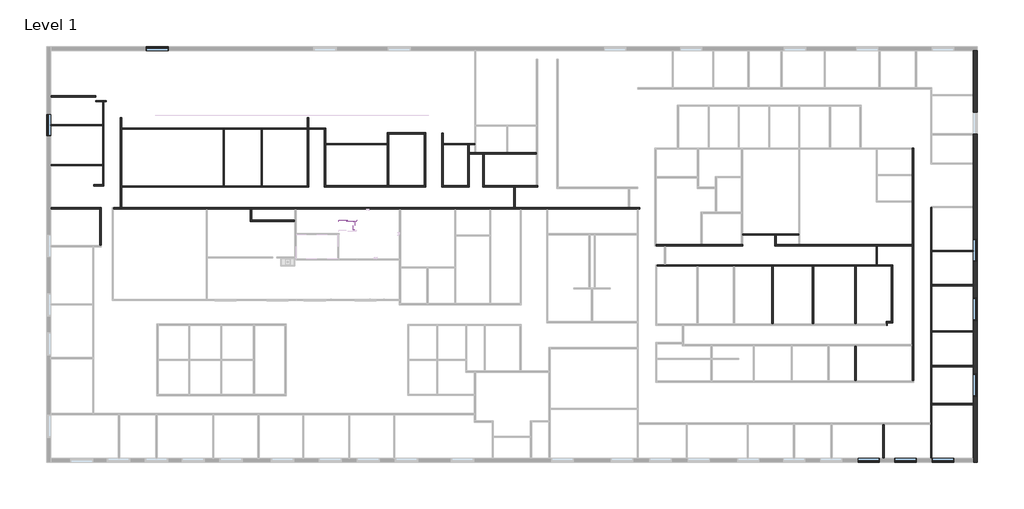
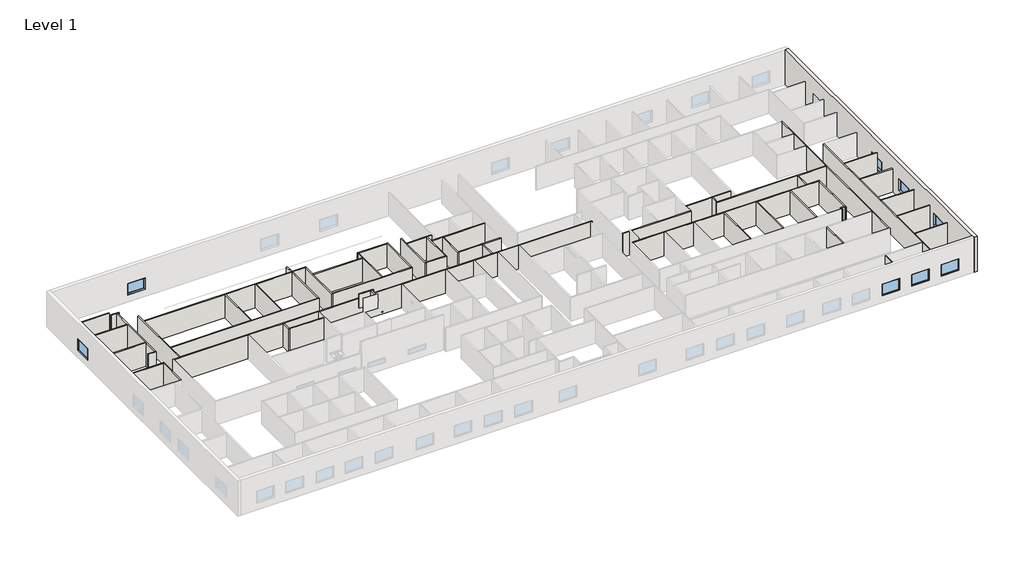
# One storey, part 3 of 4: 55 walls, 8 windows.
"""IFC4 building model written with IfcOpenShell, lengths in millimetres."""

import ifcopenshell
import ifcopenshell.guid

model = None  # the IFC model being written
_history = None  # IfcOwnerHistory: only IFC2X3 demands one
_inside = {}  # id of a spatial element -> (the spatial element, [elements in it])
_under = {}  # id of a project, library or spatial element -> (it, [spatial elements below it])
_declared = {}  # id of a project -> (the project, [libraries it declares])
_typed = {}  # id of a type object -> (the type object, [elements of that type])
_made_of = {}  # id of a material, layer set ... -> (it, [elements and type objects made of it])


def new_model(schema):
    """Start an empty IFC model of exactly this schema.

    Asked for "IFC4X3", IfcOpenShell would pick the latest addendum, in which some entities
    have other attributes; the version numbers below select the first issue.
    IFC2X3 requires an IfcOwnerHistory on every rooted entity: one is made here for all.
    """
    global model, _history
    if schema == "IFC4X3":
        model = ifcopenshell.file(schema_version=(4, 3, 0, 0))
    else:
        model = ifcopenshell.file(schema=schema)
    _inside.clear()
    _under.clear()
    _declared.clear()
    _typed.clear()
    _made_of.clear()
    _history = None
    if model.schema == "IFC2X3":
        org = make("IfcOrganization", Name="unknown")
        user = make(
            "IfcPersonAndOrganization",
            ThePerson=make("IfcPerson", FamilyName="unknown"),
            TheOrganization=org,
        )
        app = make(
            "IfcApplication",
            ApplicationDeveloper=org,
            Version="unknown",
            ApplicationFullName="unknown",
            ApplicationIdentifier="unknown",
        )
        _history = make(
            "IfcOwnerHistory",
            OwningUser=user,
            OwningApplication=app,
            ChangeAction="ADDED",
            CreationDate=0,
        )
    return model


def make(cls, **values):
    """One entity of the class cls with the attributes given. An attribute that is None is left unset."""
    return model.create_entity(
        cls, **{name: value for name, value in values.items() if value is not None}
    )


def rooted(cls, **values):
    """An entity with a GlobalId (a new one), such as an element, a storey or a relation."""
    return make(cls, GlobalId=ifcopenshell.guid.new(), OwnerHistory=_history, **values)


def si_unit(unit_type, name, prefix=None):
    """IfcSIUnit, for example si_unit("LENGTHUNIT", "METRE", prefix="MILLI")."""
    return make("IfcSIUnit", UnitType=unit_type, Prefix=prefix, Name=name)


def assignment(units):
    """IfcUnitAssignment: the units of a project."""
    return None if units is None else make("IfcUnitAssignment", Units=units)


def point(xyz):
    """IfcCartesianPoint."""
    return None if xyz is None else make("IfcCartesianPoint", Coordinates=xyz)


def direction(xyz):
    """IfcDirection."""
    return None if xyz is None else make("IfcDirection", DirectionRatios=xyz)


def frame(location, z_axis=None, x_axis=None):
    """IfcAxis2Placement3D, a coordinate frame: its origin and axes. An axis left out is left unset."""
    return make(
        "IfcAxis2Placement3D",
        Location=point(location),
        Axis=direction(z_axis),
        RefDirection=direction(x_axis),
    )


def origin():
    """The frame at (0, 0, 0) with its axes left unset."""
    return frame((0.0, 0.0, 0.0))


def origin_with_axes():
    """The frame at (0, 0, 0) with the z axis (0, 0, 1) and the x axis (1, 0, 0) written out."""
    return frame((0.0, 0.0, 0.0), z_axis=(0.0, 0.0, 1.0), x_axis=(1.0, 0.0, 0.0))


def place(relative_to, where):
    """IfcLocalPlacement: puts the frame where relative to a parent placement (None: the world)."""
    return make(
        "IfcLocalPlacement", PlacementRelTo=relative_to, RelativePlacement=where
    )


def context(
    kind, dimensions, precision=None, world=None, true_north=None, identifier=None
):
    """IfcGeometricRepresentationContext, for example the 3D "Model" context."""
    return make(
        "IfcGeometricRepresentationContext",
        ContextIdentifier=identifier,
        ContextType=kind,
        CoordinateSpaceDimension=dimensions,
        Precision=precision,
        WorldCoordinateSystem=world,
        TrueNorth=true_north,
    )


def project(units=None, contexts=None):
    """IfcProject with its units and contexts."""
    return rooted(
        "IfcProject",
        Name="project",
        RepresentationContexts=contexts,
        UnitsInContext=assignment(units),
    )


def spatial(cls, under=None, at=None, **own):
    """A site, building, storey or space (cls), placed at a placement, below another one or the project."""
    s = rooted(cls, ObjectPlacement=at, **own)
    if under is not None:
        _under.setdefault(under.id(), (under, []))[1].append(s)
    return s


def polyline(points):
    """IfcPolyline through the points."""
    return make("IfcPolyline", Points=[point(p) for p in points])


def outline(outer, holes=None, kind="AREA"):
    """IfcArbitraryClosedProfileDef: a profile drawn as a closed curve; with holes, ...WithVoids."""
    if holes is None:
        return make("IfcArbitraryClosedProfileDef", ProfileType=kind, OuterCurve=outer)
    return make(
        "IfcArbitraryProfileDefWithVoids",
        ProfileType=kind,
        OuterCurve=outer,
        InnerCurves=holes,
    )


def extrude(swept, where, along, depth):
    """IfcExtrudedAreaSolid: the profile swept, set in the frame where, extruded along a direction by depth."""
    return make(
        "IfcExtrudedAreaSolid",
        SweptArea=swept,
        Position=where,
        ExtrudedDirection=direction(along),
        Depth=depth,
    )


def faces_of(points, faces, orient=None, outer=None):
    """IfcFace entities. A face is a list of loops; a loop is a list of indices into points, from 0.

    orient and outer hold one flag for each loop. By default every Orientation is true, the
    first loop of a face is its IfcFaceOuterBound and the others are IfcFaceBound.
    """
    made = []
    for i, loops in enumerate(faces):
        bounds = []
        for j, loop in enumerate(loops):
            is_outer = j == 0 if outer is None else outer[i][j]
            bounds.append(
                make(
                    "IfcFaceOuterBound" if is_outer else "IfcFaceBound",
                    Bound=make("IfcPolyLoop", Polygon=[points[k] for k in loop]),
                    Orientation=True if orient is None else orient[i][j],
                )
            )
        made.append(make("IfcFace", Bounds=bounds))
    return made


def faceted_brep(points, faces, orient=None, outer=None, voids=None):
    """IfcFacetedBrep: a solid bounded by flat faces; with voids (closed shells), ...WithVoids."""
    shared = [point(p) for p in points]
    hull = make("IfcClosedShell", CfsFaces=faces_of(shared, faces, orient, outer))
    if voids is None:
        return make("IfcFacetedBrep", Outer=hull)
    return make(
        "IfcFacetedBrepWithVoids",
        Outer=hull,
        Voids=[
            make(cls, CfsFaces=faces_of(shared, fs, o, b)) for cls, fs, o, b in voids
        ],
    )


def shape(context_of_items, identifier, shape_type, items):
    """IfcShapeRepresentation: the items that make up one representation, for example the "Body"."""
    return make(
        "IfcShapeRepresentation",
        ContextOfItems=context_of_items,
        RepresentationIdentifier=identifier,
        RepresentationType=shape_type,
        Items=items,
    )


def source(mapping_origin, context_of_items, identifier, shape_type, items):
    """IfcRepresentationMap: a shape defined once, which mapped items show again and again."""
    return make(
        "IfcRepresentationMap",
        MappingOrigin=mapping_origin,
        MappedRepresentation=shape(context_of_items, identifier, shape_type, items),
    )


def transform(
    local_origin,
    x_axis=None,
    y_axis=None,
    z_axis=None,
    scale=None,
    scale2=None,
    scale3=None,
    uniform=True,
):
    """IfcCartesianTransformationOperator3D, or its non-uniform kind. x_axis, y_axis, z_axis: its Axis1, 2, 3."""
    if uniform:
        return make(
            "IfcCartesianTransformationOperator3D",
            Axis1=direction(x_axis),
            Axis2=direction(y_axis),
            LocalOrigin=point(local_origin),
            Scale=scale,
            Axis3=direction(z_axis),
        )
    return make(
        "IfcCartesianTransformationOperator3DnonUniform",
        Axis1=direction(x_axis),
        Axis2=direction(y_axis),
        LocalOrigin=point(local_origin),
        Scale=scale,
        Axis3=direction(z_axis),
        Scale2=scale2,
        Scale3=scale3,
    )


def mapped(mapping_source, mapping_target):
    """IfcMappedItem: shows the shape of a source again, moved by a transform."""
    return make(
        "IfcMappedItem", MappingSource=mapping_source, MappingTarget=mapping_target
    )


def made_of(thing, what):
    """Note that an element or type object is made of a material, layer set ...; save() writes the relation."""
    if what is not None:
        _made_of.setdefault(what.id(), (what, []))[1].append(thing)
    return thing


def element(
    cls,
    number,
    at=None,
    inside=None,
    cuts=None,
    type_object=None,
    material=None,
    context=None,
    identifier="Body",
    shape_type=None,
    held_by="IfcProductDefinitionShape",
    body=None,
    shapes=None,
    **own,
):
    """One element of the class cls, such as IfcWall. Its Tag is "e" and its number.

    at: its placement. inside: the storey or other place that contains it. cuts: it is an
    opening in that element (IfcRelVoidsElement). A single representation is given by context,
    identifier, shape_type and body (its items); several are given by shapes. held_by: the class
    of the entity that holds the representations. save() writes the other relations.
    """
    e = rooted(cls, Tag="e%d" % number, ObjectPlacement=at, **own)
    if body is not None:
        shapes = [shape(context, identifier, shape_type, body)]
    if shapes is not None:
        e.Representation = make(held_by, Representations=shapes)
    if inside is not None:
        _inside.setdefault(inside.id(), (inside, []))[1].append(e)
    if cuts is not None:
        rooted(
            "IfcRelVoidsElement", RelatingBuildingElement=cuts, RelatedOpeningElement=e
        )
    if type_object is not None:
        _typed.setdefault(type_object.id(), (type_object, []))[1].append(e)
    return made_of(e, material)


def aggregate(whole, parts):
    """IfcRelAggregates: a whole, such as a stair, and the parts it consists of."""
    return rooted("IfcRelAggregates", RelatingObject=whole, RelatedObjects=parts)


def save(model, path):
    """Write the relations noted so far, then the file.

    IfcRelAggregates (storeys below a building ...), IfcRelContainedInSpatialStructure (elements
    in a storey), IfcRelDefinesByType, IfcRelAssociatesMaterial and IfcRelDeclares: one each for
    every whole, place, type object, material and project.
    """
    for whole, parts in _under.values():
        aggregate(whole, parts)
    for where, things in _inside.values():
        rooted(
            "IfcRelContainedInSpatialStructure",
            RelatedElements=things,
            RelatingStructure=where,
        )
    for kind, things in _typed.values():
        rooted("IfcRelDefinesByType", RelatedObjects=things, RelatingType=kind)
    for what, things in _made_of.values():
        rooted("IfcRelAssociatesMaterial", RelatedObjects=things, RelatingMaterial=what)
    for by, libraries in _declared.values():
        rooted("IfcRelDeclares", RelatingContext=by, RelatedDefinitions=libraries)
    model.write(path)


def window_d56d71bd(model_context):
    return source(origin(), model_context, "Body", "SweptSolid", [
        extrude(outline(polyline([(990.6, 50.8), (-1066.8, 50.8), (-1066.8, 63.5), (990.6, 63.5), (990.6, 50.8)])), frame((0.0, 0.0, 977.9), z_axis=(0.0, 0.0, 1.0), x_axis=(1.0, 0.0, 0.0)), (0.0, 0.0, 1.0), 1397.0),
        extrude(outline(polyline([(2419.35, -1111.25), (933.45, -1111.25), (933.45, 1035.05), (2419.35, 1035.05), (2419.35, -1111.25)]), holes=[polyline([(2374.9, -1066.8), (2374.9, 990.6), (977.9, 990.6), (977.9, -1066.8), (2374.9, -1066.8)])]), frame((0.0, 34.925, 0.0), z_axis=(0.0, 1.0, 0.0), x_axis=(0.0, 0.0, 1.0)), (0.0, 0.0, 1.0), 44.45),
        extrude(outline(polyline([(2438.4, -1130.3), (914.4, -1130.3), (914.4, 1054.1), (2438.4, 1054.1), (2438.4, -1130.3)]), holes=[polyline([(2406.65, -1098.55), (2406.65, 1022.35), (946.15, 1022.35), (946.15, -1098.55), (2406.65, -1098.55)])]), frame((0.0, -206.375, 0.0), z_axis=(0.0, 1.0, 0.0), x_axis=(0.0, 0.0, 1.0)), (0.0, 0.0, 1.0), 241.3),
        extrude(outline(polyline([(2438.4, 1054.1), (2438.4, -1130.3), (914.4, -1130.3), (914.4, 1054.1), (2438.4, 1054.1)]), holes=[polyline([(2419.35, 1035.05), (933.45, 1035.05), (933.45, -1111.25), (2419.35, -1111.25), (2419.35, 1035.05)])]), frame((0.0, 34.925, 0.0), z_axis=(0.0, 1.0, 0.0), x_axis=(0.0, 0.0, 1.0)), (0.0, 0.0, 1.0), 171.45),
    ])


model = new_model("IFC4")

# Units and contexts
model_context = context("Model", 3, world=origin())
ifc_project = project(units=[si_unit("LENGTHUNIT", "METRE", prefix="MILLI")], contexts=[model_context])

# Site, building, storey
site = spatial("IfcSite", under=ifc_project)
building = spatial("IfcBuilding", under=site)
storey = spatial("IfcBuildingStorey", under=building, Name="Level 1", Elevation=0.0)

# Walls
placement = place(None, origin())
element("IfcWall", 1, ObjectType="Exterior Wall", at=placement, inside=storey, context=model_context, shape_type="Brep", body=[
    faceted_brep([(139716.6178914, 17535.8048706, 0.0), (139716.6178914, 6497.9173706, 0.0), (139716.6178914, 6374.0923706, 0.0), (139716.6178914, -22532.6951294, 0.0), (139716.6178914, -22945.4451294, 0.0), (139716.6178914, -22945.4451294, 4572.0), (139716.6178914, -22532.6951294, 4572.0), (139716.6178914, 17535.8048706, 4572.0), (139716.6178914, -16439.8701294, 2438.4), (139716.6178914, -16439.8701294, 914.4), (139716.6178914, -14255.4701294, 914.4), (139716.6178914, -14255.4701294, 2438.4), (139716.6178914, -8972.2701294, 2438.4), (139716.6178914, -8972.2701294, 914.4), (139716.6178914, -6787.8701294, 914.4), (139716.6178914, -6787.8701294, 2438.4), (139716.6178914, -3181.0701294, 2438.4), (139716.6178914, -3181.0701294, 914.4), (139716.6178914, -996.6701294, 914.4), (139716.6178914, -996.6701294, 2438.4), (139716.6178914, 9309.3798706, 2438.4), (139716.6178914, 9309.3798706, 914.4), (139716.6178914, 11493.7798706, 914.4), (139716.6178914, 11493.7798706, 2438.4), (140129.3678914, -22945.4451294, 0.0), (140129.3678914, 17535.8048706, 0.0), (140129.3678914, 17535.8048706, 4572.0), (140129.3678914, -22945.4451294, 4572.0), (140129.3678914, -16439.8701294, 914.4), (140129.3678914, -16439.8701294, 2438.4), (140129.3678914, -14255.4701294, 2438.4), (140129.3678914, -14255.4701294, 914.4), (140129.3678914, -8972.2701294, 914.4), (140129.3678914, -8972.2701294, 2438.4), (140129.3678914, -6787.8701294, 2438.4), (140129.3678914, -6787.8701294, 914.4), (140129.3678914, -3181.0701294, 914.4), (140129.3678914, -3181.0701294, 2438.4), (140129.3678914, -996.6701294, 2438.4), (140129.3678914, -996.6701294, 914.4), (140129.3678914, 9309.3798706, 914.4), (140129.3678914, 9309.3798706, 2438.4), (140129.3678914, 11493.7798706, 2438.4), (140129.3678914, 11493.7798706, 914.4)], [[[0, 1, 2, 3, 4, 5, 6, 7], [8, 9, 10, 11], [12, 13, 14, 15], [16, 17, 18, 19], [20, 21, 22, 23]], [[24, 25, 26, 27], [28, 29, 30, 31], [32, 33, 34, 35], [36, 37, 38, 39], [40, 41, 42, 43]], [[4, 3, 2, 1, 0, 25, 24]], [[7, 6, 5, 27, 26]], [[0, 7, 26, 25]], [[5, 4, 24, 27]], [[8, 29, 28, 9]], [[9, 28, 31, 10]], [[10, 31, 30, 11]], [[29, 8, 11, 30]], [[12, 33, 32, 13]], [[13, 32, 35, 14]], [[14, 35, 34, 15]], [[33, 12, 15, 34]], [[16, 37, 36, 17]], [[17, 36, 39, 18]], [[18, 39, 38, 19]], [[37, 16, 19, 38]], [[20, 41, 40, 21]], [[21, 40, 43, 22]], [[22, 43, 42, 23]], [[41, 20, 23, 42]]]),
])
element("IfcWall", 2, ObjectType="Interior - 4 7/8\" Partition (1-hr)", at=placement, inside=storey, context=model_context, shape_type="Brep", body=[
    faceted_brep([(54053.4683253, -1628.1381812, 0.0), (54053.4683253, 2105.6618188, 0.0), (54053.4683253, 2105.6618188, 3048.0), (54053.4683253, -1628.1381812, 3048.0), (53929.6433253, 2105.6618188, 0.0), (53929.6433253, 1981.8368188, 0.0), (53929.6433253, -1628.1381812, 0.0), (53929.6433253, -1628.1381812, 3048.0), (53929.6433253, 1981.8368188, 3048.0), (53929.6433253, 2105.6618188, 3048.0)], [[[0, 1, 2, 3]], [[4, 5, 6, 7, 8, 9]], [[1, 0, 6, 5, 4]], [[3, 2, 9, 8, 7]], [[0, 3, 7, 6]], [[2, 1, 4, 9]]]),
])
element("IfcWall", 3, ObjectType="Interior - 4 7/8\" Partition (1-hr)", at=placement, inside=storey, context=model_context, shape_type="SweptSolid", body=[
    extrude(outline(polyline([(49102.1178914, 2105.6618188), (53929.6433253, 2105.6618188), (53929.6433253, 1981.8368188), (49102.1178914, 1981.8368188), (49102.1178914, 2105.6618188)])), origin_with_axes(), (0.0, 0.0, 1.0), 3048.0),
])
element("IfcWall", 4, ObjectType="Interior - 4 7/8\" Partition (1-hr)", at=placement, inside=storey, context=model_context, shape_type="Brep", body=[
    faceted_brep([(55252.655131, 1981.8368188, 0.0), (64363.2514852, 1981.8368188, 0.0), (64487.0764852, 1981.8368188, 0.0), (68717.830131, 1981.8368188, 0.0), (68841.655131, 1981.8368188, 0.0), (73075.4514852, 1981.8368188, 0.0), (73199.2764852, 1981.8368188, 0.0), (83337.0514852, 1981.8368188, 0.0), (83460.8764852, 1981.8368188, 0.0), (95198.8514852, 1981.8368188, 0.0), (95322.6764852, 1981.8368188, 0.0), (106944.7639852, 1981.8368188, 0.0), (106944.7639852, 1981.8368188, 3048.0), (95322.6764852, 1981.8368188, 3048.0), (95198.8514852, 1981.8368188, 3048.0), (83460.8764852, 1981.8368188, 3048.0), (83337.0514852, 1981.8368188, 3048.0), (73199.2764852, 1981.8368188, 3048.0), (73075.4514852, 1981.8368188, 3048.0), (68841.655131, 1981.8368188, 3048.0), (68717.830131, 1981.8368188, 3048.0), (64487.0764852, 1981.8368188, 3048.0), (64363.2514852, 1981.8368188, 3048.0), (55252.655131, 1981.8368188, 3048.0), (106944.7639852, 2105.6618188, 0.0), (56065.455131, 2105.6618188, 0.0), (55941.630131, 2105.6618188, 0.0), (55252.655131, 2105.6618188, 0.0), (55252.655131, 2105.6618188, 3048.0), (55941.630131, 2105.6618188, 3048.0), (56065.455131, 2105.6618188, 3048.0), (106944.7639852, 2105.6618188, 3048.0)], [[[0, 1, 2, 3, 4, 5, 6, 7, 8, 9, 10, 11, 12, 13, 14, 15, 16, 17, 18, 19, 20, 21, 22, 23]], [[24, 25, 26, 27, 28, 29, 30, 31]], [[11, 10, 9, 8, 7, 6, 5, 4, 3, 2, 1, 0, 27, 26, 25, 24]], [[12, 11, 24, 31]], [[23, 22, 21, 20, 19, 18, 17, 16, 15, 14, 13, 12, 31, 30, 29, 28]], [[0, 23, 28, 27]]]),
])
element("IfcWall", 5, ObjectType="Interior - 4 7/8\" Partition (1-hr)", at=placement, inside=storey, context=model_context, shape_type="Brep", body=[
    faceted_brep([(54320.2303914, 4363.6075038, 0.0), (54320.2303914, 12510.9870321, 0.0), (54320.2303914, 12510.9870321, 3048.0), (54320.2303914, 4363.6075038, 3048.0), (54196.4053914, 12510.9870321, 0.0), (54196.4053914, 10272.6120321, 0.0), (54196.4053914, 10148.7870321, 0.0), (54196.4053914, 6345.9759689, 0.0), (54196.4053914, 6222.1509689, 0.0), (54196.4053914, 4363.6075038, 0.0), (54196.4053914, 4363.6075038, 3048.0), (54196.4053914, 6222.1509689, 3048.0), (54196.4053914, 6345.9759689, 3048.0), (54196.4053914, 10148.7870321, 3048.0), (54196.4053914, 10272.6120321, 3048.0), (54196.4053914, 12510.9870321, 3048.0)], [[[0, 1, 2, 3]], [[4, 5, 6, 7, 8, 9, 10, 11, 12, 13, 14, 15]], [[1, 0, 9, 8, 7, 6, 5, 4]], [[3, 2, 15, 14, 13, 12, 11, 10]], [[0, 3, 10, 9]], [[2, 1, 4, 15]]]),
])
element("IfcWall", 6, ObjectType="Interior - 4 7/8\" Partition (1-hr)", at=placement, inside=storey, context=model_context, shape_type="Brep", body=[
    faceted_brep([(54559.8105998, 12634.8120321, 0.0), (53543.8105998, 12634.8120321, 0.0), (53543.8105998, 12634.8120321, 3048.0), (54559.8105998, 12634.8120321, 3048.0), (54559.8105998, 12510.9870321, 0.0), (54559.8105998, 12510.9870321, 3048.0), (54320.2303914, 12510.9870321, 3048.0), (54196.4053914, 12510.9870321, 3048.0), (53543.8105998, 12510.9870321, 3048.0), (53543.8105998, 12510.9870321, 0.0), (54196.4053914, 12510.9870321, 0.0), (54320.2303914, 12510.9870321, 0.0)], [[[0, 1, 2, 3]], [[4, 5, 6, 7, 8, 9, 10, 11]], [[1, 0, 4, 11, 10, 9]], [[2, 1, 9, 8]], [[3, 2, 8, 7, 6, 5]], [[0, 3, 5, 4]]]),
])
element("IfcWall", 7, ObjectType="Interior - 4 7/8\" Partition (1-hr)", at=placement, inside=storey, context=model_context, shape_type="SweptSolid", body=[
    extrude(outline(polyline([(49102.1178914, 13092.0120321), (53543.8105998, 13092.0120321), (53543.8105998, 12968.1870321), (49102.1178914, 12968.1870321), (49102.1178914, 13092.0120321)])), origin_with_axes(), (0.0, 0.0, 1.0), 3048.0),
])
element("IfcWall", 8, ObjectType="Interior - 4 7/8\" Partition (1-hr)", at=placement, inside=storey, context=model_context, shape_type="SweptSolid", body=[
    extrude(outline(polyline([(49102.1178914, 10272.6120321), (54196.4053914, 10272.6120321), (54196.4053914, 10148.7870321), (49102.1178914, 10148.7870321), (49102.1178914, 10272.6120321)])), origin_with_axes(), (0.0, 0.0, 1.0), 3048.0),
])
element("IfcWall", 9, ObjectType="Interior - 4 7/8\" Partition (1-hr)", at=placement, inside=storey, context=model_context, shape_type="SweptSolid", body=[
    extrude(outline(polyline([(49102.1178914, 6345.9759689), (54196.4053914, 6345.9759689), (54196.4053914, 6222.1509689), (49102.1178914, 6222.1509689), (49102.1178914, 6345.9759689)])), origin_with_axes(), (0.0, 0.0, 1.0), 3048.0),
])
element("IfcWall", 10, ObjectType="Interior - 4 7/8\" Partition (1-hr)", at=placement, inside=storey, context=model_context, shape_type="Brep", body=[
    faceted_brep([(56065.455131, 2105.6618188, 0.0), (56065.455131, 4115.4368188, 0.0), (56065.455131, 4239.2618188, 0.0), (56065.455131, 9818.5870321, 0.0), (56065.455131, 9942.4120321, 0.0), (56065.455131, 10964.580131, 0.0), (56065.455131, 10964.580131, 3048.0), (56065.455131, 9942.4120321, 3048.0), (56065.455131, 9818.5870321, 3048.0), (56065.455131, 4239.2618188, 3048.0), (56065.455131, 4115.4368188, 3048.0), (56065.455131, 2105.6618188, 3048.0), (55941.630131, 10964.580131, 0.0), (55941.630131, 2105.6618188, 0.0), (55941.630131, 2105.6618188, 3048.0), (55941.630131, 10964.580131, 3048.0)], [[[0, 1, 2, 3, 4, 5, 6, 7, 8, 9, 10, 11]], [[12, 13, 14, 15]], [[5, 4, 3, 2, 1, 0, 13, 12]], [[6, 5, 12, 15]], [[11, 10, 9, 8, 7, 6, 15, 14]], [[0, 11, 14, 13]]]),
])
element("IfcWall", 11, ObjectType="Interior - 4 7/8\" Partition (1-hr)", at=placement, inside=storey, context=model_context, shape_type="Brep", body=[
    faceted_brep([(56065.455131, 9818.5870321, 0.0), (66025.430131, 9818.5870321, 0.0), (66149.255131, 9818.5870321, 0.0), (69759.230131, 9818.5870321, 0.0), (69883.055131, 9818.5870321, 0.0), (74305.830131, 9818.5870321, 0.0), (74429.655131, 9818.5870321, 0.0), (75982.230131, 9818.5870321, 0.0), (76106.055131, 9818.5870321, 0.0), (76106.055131, 9818.5870321, 3048.0), (75982.230131, 9818.5870321, 3048.0), (74429.655131, 9818.5870321, 3048.0), (74305.830131, 9818.5870321, 3048.0), (69883.055131, 9818.5870321, 3048.0), (69759.230131, 9818.5870321, 3048.0), (66149.255131, 9818.5870321, 3048.0), (66025.430131, 9818.5870321, 3048.0), (56065.455131, 9818.5870321, 3048.0), (76106.055131, 9942.4120321, 0.0), (74429.655131, 9942.4120321, 0.0), (74305.830131, 9942.4120321, 0.0), (56065.455131, 9942.4120321, 0.0), (56065.455131, 9942.4120321, 3048.0), (74305.830131, 9942.4120321, 3048.0), (74429.655131, 9942.4120321, 3048.0), (76106.055131, 9942.4120321, 3048.0)], [[[0, 1, 2, 3, 4, 5, 6, 7, 8, 9, 10, 11, 12, 13, 14, 15, 16, 17]], [[18, 19, 20, 21, 22, 23, 24, 25]], [[8, 7, 6, 5, 4, 3, 2, 1, 0, 21, 20, 19, 18]], [[17, 16, 15, 14, 13, 12, 11, 10, 9, 25, 24, 23, 22]], [[0, 17, 22, 21]], [[9, 8, 18, 25]]]),
])
element("IfcWall", 12, ObjectType="Interior - 4 7/8\" Partition (1-hr)", at=placement, inside=storey, context=model_context, shape_type="Brep", body=[
    faceted_brep([(75982.230131, 9818.5870321, 0.0), (75982.230131, 4129.995756, 0.0), (75982.230131, 4129.995756, 3048.0), (75982.230131, 9818.5870321, 3048.0), (76106.055131, 9818.5870321, 0.0), (76106.055131, 9818.5870321, 3048.0), (76106.055131, 8419.420756, 3048.0), (76106.055131, 8295.595756, 3048.0), (76106.055131, 4253.820756, 3048.0), (76106.055131, 4129.995756, 3048.0), (76106.055131, 4129.995756, 0.0), (76106.055131, 4253.820756, 0.0), (76106.055131, 8295.595756, 0.0), (76106.055131, 8419.420756, 0.0)], [[[0, 1, 2, 3]], [[4, 5, 6, 7, 8, 9, 10, 11, 12, 13]], [[1, 0, 4, 13, 12, 11, 10]], [[3, 2, 9, 8, 7, 6, 5]], [[0, 3, 5, 4]], [[2, 1, 10, 9]]]),
])
element("IfcWall", 13, ObjectType="Interior - 4 7/8\" Partition (1-hr)", at=placement, inside=storey, context=model_context, shape_type="Brep", body=[
    faceted_brep([(76106.055131, 4129.995756, 0.0), (85935.855131, 4129.995756, 0.0), (85935.855131, 4129.995756, 3048.0), (76106.055131, 4129.995756, 3048.0), (85935.855131, 4253.820756, 0.0), (85812.030131, 4253.820756, 0.0), (82303.655131, 4253.820756, 0.0), (82179.830131, 4253.820756, 0.0), (76106.055131, 4253.820756, 0.0), (76106.055131, 4253.820756, 3048.0), (82179.830131, 4253.820756, 3048.0), (82303.655131, 4253.820756, 3048.0), (85812.030131, 4253.820756, 3048.0), (85935.855131, 4253.820756, 3048.0)], [[[0, 1, 2, 3]], [[4, 5, 6, 7, 8, 9, 10, 11, 12, 13]], [[1, 0, 8, 7, 6, 5, 4]], [[3, 2, 13, 12, 11, 10, 9]], [[0, 3, 9, 8]], [[2, 1, 4, 13]]]),
])
element("IfcWall", 14, ObjectType="Interior - 4 7/8\" Partition (1-hr)", at=placement, inside=storey, context=model_context, shape_type="Brep", body=[
    faceted_brep([(85935.855131, 4253.820756, 0.0), (85935.855131, 9460.820756, 0.0), (85935.855131, 9460.820756, 3048.0), (85935.855131, 4253.820756, 3048.0), (85812.030131, 4253.820756, 0.0), (85812.030131, 4253.820756, 3048.0), (85812.030131, 9336.995756, 3048.0), (85812.030131, 9460.820756, 3048.0), (85812.030131, 9460.820756, 0.0), (85812.030131, 9336.995756, 0.0)], [[[0, 1, 2, 3]], [[4, 5, 6, 7, 8, 9]], [[1, 0, 4, 9, 8]], [[3, 2, 7, 6, 5]], [[0, 3, 5, 4]], [[2, 1, 8, 7]]]),
])
element("IfcWall", 15, ObjectType="Interior - 4 7/8\" Partition (1-hr)", at=placement, inside=storey, context=model_context, shape_type="Brep", body=[
    faceted_brep([(85812.030131, 9460.820756, 0.0), (82179.830131, 9460.820756, 0.0), (82179.830131, 9460.820756, 3048.0), (85812.030131, 9460.820756, 3048.0), (82179.830131, 9336.995756, 0.0), (82303.655131, 9336.995756, 0.0), (85812.030131, 9336.995756, 0.0), (85812.030131, 9336.995756, 3048.0), (82303.655131, 9336.995756, 3048.0), (82179.830131, 9336.995756, 3048.0)], [[[0, 1, 2, 3]], [[4, 5, 6, 7, 8, 9]], [[1, 0, 6, 5, 4]], [[3, 2, 9, 8, 7]], [[0, 3, 7, 6]], [[2, 1, 4, 9]]]),
])
element("IfcWall", 16, ObjectType="Interior - 4 7/8\" Partition (1-hr)", at=placement, inside=storey, context=model_context, shape_type="Brep", body=[
    faceted_brep([(82179.830131, 9336.995756, 0.0), (82179.830131, 8419.420756, 0.0), (82179.830131, 8295.595756, 0.0), (82179.830131, 4253.820756, 0.0), (82179.830131, 4253.820756, 3048.0), (82179.830131, 8295.595756, 3048.0), (82179.830131, 8419.420756, 3048.0), (82179.830131, 9336.995756, 3048.0), (82303.655131, 9336.995756, 0.0), (82303.655131, 9336.995756, 3048.0), (82303.655131, 4253.820756, 3048.0), (82303.655131, 4253.820756, 0.0)], [[[0, 1, 2, 3, 4, 5, 6, 7]], [[8, 9, 10, 11]], [[3, 2, 1, 0, 8, 11]], [[7, 6, 5, 4, 10, 9]], [[0, 7, 9, 8]], [[4, 3, 11, 10]]]),
])
element("IfcWall", 17, ObjectType="Interior - 4 7/8\" Partition (1-hr)", at=placement, inside=storey, context=model_context, shape_type="SweptSolid", body=[
    extrude(outline(polyline([(76106.055131, 8419.420756), (82179.830131, 8419.420756), (82179.830131, 8295.595756), (76106.055131, 8295.595756), (76106.055131, 8419.420756)])), origin_with_axes(), (0.0, 0.0, 1.0), 3048.0),
])
element("IfcWall", 18, ObjectType="Interior - 4 7/8\" Partition (1-hr)", at=placement, inside=storey, context=model_context, shape_type="Brep", body=[
    faceted_brep([(87533.1447144, 9438.5296102, 0.0), (87533.1447144, 4129.995756, 0.0), (87533.1447144, 4129.995756, 3048.0), (87533.1447144, 9438.5296102, 3048.0), (87656.9697144, 9438.5296102, 0.0), (87656.9697144, 9438.5296102, 3048.0), (87656.9697144, 8419.420756, 3048.0), (87656.9697144, 8295.595756, 3048.0), (87656.9697144, 4253.820756, 3048.0), (87656.9697144, 4129.995756, 3048.0), (87656.9697144, 4129.995756, 0.0), (87656.9697144, 4253.820756, 0.0), (87656.9697144, 8295.595756, 0.0), (87656.9697144, 8419.420756, 0.0)], [[[0, 1, 2, 3]], [[4, 5, 6, 7, 8, 9, 10, 11, 12, 13]], [[1, 0, 4, 13, 12, 11, 10]], [[3, 2, 9, 8, 7, 6, 5]], [[0, 3, 5, 4]], [[2, 1, 10, 9]]]),
])
element("IfcWall", 19, ObjectType="Interior - 4 7/8\" Partition (1-hr)", at=placement, inside=storey, context=model_context, shape_type="Brep", body=[
    faceted_brep([(87656.9697144, 4129.995756, 0.0), (90196.9697144, 4129.995756, 0.0), (90196.9697144, 4129.995756, 3048.0), (87656.9697144, 4129.995756, 3048.0), (87656.9697144, 4253.820756, 0.0), (87656.9697144, 4253.820756, 3048.0), (90073.1447144, 4253.820756, 3048.0), (90196.9697144, 4253.820756, 3048.0), (90196.9697144, 4253.820756, 0.0), (90073.1447144, 4253.820756, 0.0)], [[[0, 1, 2, 3]], [[4, 5, 6, 7, 8, 9]], [[1, 0, 4, 9, 8]], [[3, 2, 7, 6, 5]], [[0, 3, 5, 4]], [[2, 1, 8, 7]]]),
])
element("IfcWall", 20, ObjectType="Interior - 4 7/8\" Partition (1-hr)", at=placement, inside=storey, context=model_context, shape_type="Brep", body=[
    faceted_brep([(90196.9697144, 4253.820756, 0.0), (90196.9697144, 7390.0923706, 0.0), (90196.9697144, 7513.9173706, 0.0), (90196.9697144, 8295.595756, 0.0), (90196.9697144, 8295.595756, 3048.0), (90196.9697144, 7513.9173706, 3048.0), (90196.9697144, 7390.0923706, 3048.0), (90196.9697144, 4253.820756, 3048.0), (90073.1447144, 4253.820756, 0.0), (90073.1447144, 4253.820756, 3048.0), (90073.1447144, 8295.595756, 3048.0), (90073.1447144, 8295.595756, 0.0)], [[[0, 1, 2, 3, 4, 5, 6, 7]], [[8, 9, 10, 11]], [[3, 2, 1, 0, 8, 11]], [[7, 6, 5, 4, 10, 9]], [[0, 7, 9, 8]], [[4, 3, 11, 10]]]),
])
element("IfcWall", 21, ObjectType="Interior - 4 7/8\" Partition (1-hr)", at=placement, inside=storey, context=model_context, shape_type="Brep", body=[
    faceted_brep([(87656.9697144, 8295.595756, 0.0), (90073.1447144, 8295.595756, 0.0), (90196.9697144, 8295.595756, 0.0), (90729.1866283, 8295.595756, 0.0), (90729.1866283, 8295.595756, 3048.0), (90196.9697144, 8295.595756, 3048.0), (90073.1447144, 8295.595756, 3048.0), (87656.9697144, 8295.595756, 3048.0), (87656.9697144, 8419.420756, 0.0), (87656.9697144, 8419.420756, 3048.0), (90729.1866283, 8419.420756, 3048.0), (90729.1866283, 8419.420756, 0.0)], [[[0, 1, 2, 3, 4, 5, 6, 7]], [[8, 9, 10, 11]], [[3, 2, 1, 0, 8, 11]], [[7, 6, 5, 4, 10, 9]], [[0, 7, 9, 8]], [[4, 3, 11, 10]]]),
])
element("IfcWall", 22, ObjectType="Interior - 4 7/8\" Partition (1-hr)", at=placement, inside=storey, context=model_context, shape_type="Brep", body=[
    faceted_brep([(96810.8991283, 7513.9173706, 0.0), (94002.6116283, 7513.9173706, 0.0), (93878.7866283, 7513.9173706, 0.0), (90853.0116283, 7513.9173706, 0.0), (90729.1866283, 7513.9173706, 0.0), (90196.9697144, 7513.9173706, 0.0), (90196.9697144, 7513.9173706, 3048.0), (90729.1866283, 7513.9173706, 3048.0), (90853.0116283, 7513.9173706, 3048.0), (93878.7866283, 7513.9173706, 3048.0), (94002.6116283, 7513.9173706, 3048.0), (96810.8991283, 7513.9173706, 3048.0), (96810.8991283, 7390.0923706, 0.0), (96810.8991283, 7390.0923706, 3048.0), (91665.8116283, 7390.0923706, 3048.0), (91541.9866283, 7390.0923706, 3048.0), (90196.9697144, 7390.0923706, 3048.0), (90196.9697144, 7390.0923706, 0.0), (91541.9866283, 7390.0923706, 0.0), (91665.8116283, 7390.0923706, 0.0)], [[[0, 1, 2, 3, 4, 5, 6, 7, 8, 9, 10, 11]], [[12, 13, 14, 15, 16, 17, 18, 19]], [[5, 4, 3, 2, 1, 0, 12, 19, 18, 17]], [[11, 10, 9, 8, 7, 6, 16, 15, 14, 13]], [[6, 5, 17, 16]], [[0, 11, 13, 12]]]),
])
element("IfcWall", 23, ObjectType="Interior - 4 7/8\" Partition (1-hr)", at=placement, inside=storey, context=model_context, shape_type="Brep", body=[
    faceted_brep([(91541.9866283, 7390.0923706, 0.0), (91541.9866283, 4129.995756, 0.0), (91541.9866283, 4129.995756, 3048.0), (91541.9866283, 7390.0923706, 3048.0), (91665.8116283, 7390.0923706, 0.0), (91665.8116283, 7390.0923706, 3048.0), (91665.8116283, 4253.820756, 3048.0), (91665.8116283, 4129.995756, 3048.0), (91665.8116283, 4129.995756, 0.0), (91665.8116283, 4253.820756, 0.0)], [[[0, 1, 2, 3]], [[4, 5, 6, 7, 8, 9]], [[1, 0, 4, 9, 8]], [[3, 2, 7, 6, 5]], [[0, 3, 5, 4]], [[2, 1, 8, 7]]]),
])
element("IfcWall", 24, ObjectType="Interior - 4 7/8\" Partition (1-hr)", at=placement, inside=storey, context=model_context, shape_type="Brep", body=[
    faceted_brep([(91665.8116283, 4129.995756, 0.0), (96934.7241283, 4129.995756, 0.0), (96934.7241283, 4129.995756, 3048.0), (91665.8116283, 4129.995756, 3048.0), (91665.8116283, 4253.820756, 0.0), (91665.8116283, 4253.820756, 3048.0), (96810.8991283, 4253.820756, 3048.0), (96934.7241283, 4253.820756, 3048.0), (96934.7241283, 4253.820756, 0.0), (96810.8991283, 4253.820756, 0.0)], [[[0, 1, 2, 3]], [[4, 5, 6, 7, 8, 9]], [[1, 0, 4, 9, 8]], [[3, 2, 7, 6, 5]], [[0, 3, 5, 4]], [[2, 1, 8, 7]]]),
])
element("IfcWall", 25, ObjectType="Interior - 4 7/8\" Partition (1-hr)", at=placement, inside=storey, context=model_context, shape_type="Brep", body=[
    faceted_brep([(56065.455131, 4115.4368188, 0.0), (74429.655131, 4115.4368188, 0.0), (74429.655131, 4115.4368188, 3048.0), (56065.455131, 4115.4368188, 3048.0), (74429.655131, 4239.2618188, 0.0), (74305.830131, 4239.2618188, 0.0), (69883.055131, 4239.2618188, 0.0), (69759.230131, 4239.2618188, 0.0), (66149.255131, 4239.2618188, 0.0), (66025.430131, 4239.2618188, 0.0), (56065.455131, 4239.2618188, 0.0), (56065.455131, 4239.2618188, 3048.0), (66025.430131, 4239.2618188, 3048.0), (66149.255131, 4239.2618188, 3048.0), (69759.230131, 4239.2618188, 3048.0), (69883.055131, 4239.2618188, 3048.0), (74305.830131, 4239.2618188, 3048.0), (74429.655131, 4239.2618188, 3048.0)], [[[0, 1, 2, 3]], [[4, 5, 6, 7, 8, 9, 10, 11, 12, 13, 14, 15, 16, 17]], [[1, 0, 10, 9, 8, 7, 6, 5, 4]], [[3, 2, 17, 16, 15, 14, 13, 12, 11]], [[2, 1, 4, 17]], [[0, 3, 11, 10]]]),
])
element("IfcWall", 26, ObjectType="Interior - 4 7/8\" Partition (1-hr)", at=placement, inside=storey, context=model_context, shape_type="SweptSolid", body=[
    extrude(outline(polyline([(74305.830131, 10959.1493188), (74429.655131, 10959.1493188), (74429.655131, 9942.4120321), (74305.830131, 9942.4120321), (74305.830131, 10959.1493188)])), origin_with_axes(), (0.0, 0.0, 1.0), 3048.0),
    extrude(outline(polyline([(74429.655131, 4239.2618188), (74305.830131, 4239.2618188), (74305.830131, 9818.5870321), (74429.655131, 9818.5870321), (74429.655131, 4239.2618188)])), origin_with_axes(), (0.0, 0.0, 1.0), 3048.0),
])
element("IfcWall", 27, ObjectType="Interior - 4 7/8\" Partition (1-hr)", at=placement, inside=storey, context=model_context, shape_type="SweptSolid", body=[
    extrude(outline(polyline([(69883.055131, 9818.5870321), (69883.055131, 4239.2618188), (69759.230131, 4239.2618188), (69759.230131, 9818.5870321), (69883.055131, 9818.5870321)])), origin_with_axes(), (0.0, 0.0, 1.0), 3048.0),
])
element("IfcWall", 28, ObjectType="Interior - 4 7/8\" Partition (1-hr)", at=placement, inside=storey, context=model_context, shape_type="SweptSolid", body=[
    extrude(outline(polyline([(66025.430131, 4239.2618188), (66025.430131, 9818.5870321), (66149.255131, 9818.5870321), (66149.255131, 4239.2618188), (66025.430131, 4239.2618188)])), origin_with_axes(), (0.0, 0.0, 1.0), 3048.0),
])
element("IfcWall", 29, ObjectType="Interior - 4 7/8\" Partition (1-hr)", at=placement, inside=storey, context=model_context, shape_type="Brep", body=[
    faceted_brep([(68717.830131, 1981.8368188, 0.0), (68717.830131, 762.6368188, 0.0), (68717.830131, 762.6368188, 3048.0), (68717.830131, 1981.8368188, 3048.0), (68841.655131, 1981.8368188, 0.0), (68841.655131, 1981.8368188, 3048.0), (68841.655131, 886.4618188, 3048.0), (68841.655131, 762.6368188, 3048.0), (68841.655131, 762.6368188, 0.0), (68841.655131, 886.4618188, 0.0)], [[[0, 1, 2, 3]], [[4, 5, 6, 7, 8, 9]], [[1, 0, 4, 9, 8]], [[3, 2, 7, 6, 5]], [[2, 1, 8, 7]], [[0, 3, 5, 4]]]),
])
element("IfcWall", 30, ObjectType="Interior - 4 7/8\" Partition (1-hr)", at=placement, inside=storey, context=model_context, shape_type="SweptSolid", body=[
    extrude(outline(polyline([(73075.4514852, 762.6368188), (68841.655131, 762.6368188), (68841.655131, 886.4618188), (73075.4514852, 886.4618188), (73075.4514852, 762.6368188)])), origin_with_axes(), (0.0, 0.0, 1.0), 3048.0),
])
element("IfcWall", 31, ObjectType="Interior - 4 7/8\" Partition (1-hr)", at=placement, inside=storey, context=model_context, shape_type="Brep", body=[
    faceted_brep([(53343.9178914, 4239.7825038, 0.0), (54320.2303914, 4239.7825038, 0.0), (54320.2303914, 4239.7825038, 3048.0), (53343.9178914, 4239.7825038, 3048.0), (53343.9178914, 4363.6075038, 0.0), (53343.9178914, 4363.6075038, 3048.0), (54196.4053914, 4363.6075038, 3048.0), (54320.2303914, 4363.6075038, 3048.0), (54320.2303914, 4363.6075038, 0.0), (54196.4053914, 4363.6075038, 0.0)], [[[0, 1, 2, 3]], [[4, 5, 6, 7, 8, 9]], [[1, 0, 4, 9, 8]], [[3, 2, 7, 6, 5]], [[0, 3, 5, 4]], [[2, 1, 8, 7]]]),
])
element("IfcWall", 32, ObjectType="Interior - 4 7/8\" Partition (1-hr)", at=placement, inside=storey, context=model_context, shape_type="Brep", body=[
    faceted_brep([(77415.6764852, 762.6368188, 2743.2), (78815.8514852, 762.6368188, 2743.2), (78939.6764852, 762.6368188, 2743.2), (79182.5639852, 762.6368188, 2743.2), (79182.5639852, 762.6368188, 4572.0), (78939.6764852, 762.6368188, 4572.0), (78815.8514852, 762.6368188, 4572.0), (77415.6764852, 762.6368188, 4572.0), (77415.6764852, 886.4618188, 2743.2), (77415.6764852, 886.4618188, 4572.0), (79182.5639852, 886.4618188, 4572.0), (79182.5639852, 886.4618188, 2743.2)], [[[0, 1, 2, 3, 4, 5, 6, 7]], [[8, 9, 10, 11]], [[3, 2, 1, 0, 8, 11]], [[4, 3, 11, 10]], [[7, 6, 5, 4, 10, 9]], [[0, 7, 9, 8]]]),
])
element("IfcWall", 33, ObjectType="Interior - 4 7/8\" Partition (1-hr)", at=placement, inside=storey, context=model_context, shape_type="SweptSolid", body=[
    extrude(outline(polyline([(78815.8514852, -110.8239048), (78815.8514852, 762.6368188), (78939.6764852, 762.6368188), (78939.6764852, -110.8239048), (78815.8514852, -110.8239048)])), frame((0.0, 0.0, 2743.2), z_axis=(0.0, 0.0, 1.0), x_axis=(1.0, 0.0, 0.0)), (0.0, 0.0, 1.0), 1828.8),
])
element("IfcWall", 34, ObjectType="Interior - 4 7/8\" Partition (1-hr)", at=placement, inside=storey, context=model_context, shape_type="Brep", body=[
    faceted_brep([(133865.8936489, -14951.2015997, 0.0), (133865.8936489, 7963.1798706, 0.0), (133865.8936489, 7963.1798706, 3048.0), (133865.8936489, -14951.2015997, 3048.0), (133742.0686489, -14951.2015997, 0.0), (133742.0686489, -14951.2015997, 3048.0), (133742.0686489, -11468.2265997, 3048.0), (133742.0686489, -11344.4015997, 3048.0), (133742.0686489, -1663.8265997, 3048.0), (133742.0686489, -1540.0015997, 3048.0), (133742.0686489, 2636.5588328, 3048.0), (133742.0686489, 2760.3838328, 3048.0), (133742.0686489, 5237.9568517, 3048.0), (133742.0686489, 5361.7818517, 3048.0), (133742.0686489, 7839.3548706, 3048.0), (133742.0686489, 7963.1798706, 3048.0), (133742.0686489, 7963.1798706, 0.0), (133742.0686489, 7839.3548706, 0.0), (133742.0686489, 5361.7818517, 0.0), (133742.0686489, 5237.9568517, 0.0), (133742.0686489, 2760.3838328, 0.0), (133742.0686489, 2636.5588328, 0.0), (133742.0686489, -1540.0015997, 0.0), (133742.0686489, -1663.8265997, 0.0), (133742.0686489, -11344.4015997, 0.0), (133742.0686489, -11468.2265997, 0.0)], [[[0, 1, 2, 3]], [[4, 5, 6, 7, 8, 9, 10, 11, 12, 13, 14, 15, 16, 17, 18, 19, 20, 21, 22, 23, 24, 25]], [[1, 0, 4, 25, 24, 23, 22, 21, 20, 19, 18, 17, 16]], [[3, 2, 15, 14, 13, 12, 11, 10, 9, 8, 7, 6, 5]], [[0, 3, 5, 4]], [[2, 1, 16, 15]]]),
])
element("IfcWall", 35, ObjectType="Interior - 4 7/8\" Partition (1-hr)", at=placement, inside=storey, context=model_context, shape_type="Brep", body=[
    faceted_brep([(108567.4936489, -1663.8265997, 0.0), (117051.0936489, -1663.8265997, 0.0), (117051.0936489, -1663.8265997, 3048.0), (108567.4936489, -1663.8265997, 3048.0), (108567.4936489, -1540.0015997, 0.0), (108567.4936489, -1540.0015997, 3048.0), (112970.7155477, -1540.0015997, 3048.0), (113094.5405477, -1540.0015997, 3048.0), (116927.2686489, -1540.0015997, 3048.0), (117051.0936489, -1540.0015997, 3048.0), (117051.0936489, -1540.0015997, 0.0), (116927.2686489, -1540.0015997, 0.0), (113094.5405477, -1540.0015997, 0.0), (112970.7155477, -1540.0015997, 0.0)], [[[0, 1, 2, 3]], [[4, 5, 6, 7, 8, 9, 10, 11, 12, 13]], [[1, 0, 4, 13, 12, 11, 10]], [[3, 2, 9, 8, 7, 6, 5]], [[0, 3, 5, 4]], [[2, 1, 10, 9]]]),
])
element("IfcWall", 36, ObjectType="Interior - 4 7/8\" Partition (1-hr)", at=placement, inside=storey, context=model_context, shape_type="Brep", body=[
    faceted_brep([(135520.4991283, 2092.6048706, 0.0), (135520.4991283, -19067.1826294, 0.0), (135520.4991283, -19191.0076294, 0.0), (135520.4991283, -22532.6951294, 0.0), (135520.4991283, -22532.6951294, 3048.0), (135520.4991283, -19191.0076294, 3048.0), (135520.4991283, -19067.1826294, 3048.0), (135520.4991283, 2092.6048706, 3048.0), (135644.3241283, 2092.6048706, 0.0), (135644.3241283, 2092.6048706, 3048.0), (135644.3241283, -2098.8015997, 3048.0), (135644.3241283, -2222.6265997, 3048.0), (135644.3241283, -5468.5914836, 3048.0), (135644.3241283, -5592.4164836, 3048.0), (135644.3241283, -9997.5305461, 3048.0), (135644.3241283, -10121.3555461, 3048.0), (135644.3241283, -13417.4024211, 3048.0), (135644.3241283, -13541.2274211, 3048.0), (135644.3241283, -17162.1826294, 3048.0), (135644.3241283, -17286.0076294, 3048.0), (135644.3241283, -22532.6951294, 3048.0), (135644.3241283, -22532.6951294, 0.0), (135644.3241283, -17286.0076294, 0.0), (135644.3241283, -17162.1826294, 0.0), (135644.3241283, -13541.2274211, 0.0), (135644.3241283, -13417.4024211, 0.0), (135644.3241283, -10121.3555461, 0.0), (135644.3241283, -9997.5305461, 0.0), (135644.3241283, -5592.4164836, 0.0), (135644.3241283, -5468.5914836, 0.0), (135644.3241283, -2222.6265997, 0.0), (135644.3241283, -2098.8015997, 0.0)], [[[0, 1, 2, 3, 4, 5, 6, 7]], [[8, 9, 10, 11, 12, 13, 14, 15, 16, 17, 18, 19, 20, 21, 22, 23, 24, 25, 26, 27, 28, 29, 30, 31]], [[3, 2, 1, 0, 8, 31, 30, 29, 28, 27, 26, 25, 24, 23, 22, 21]], [[7, 6, 5, 4, 20, 19, 18, 17, 16, 15, 14, 13, 12, 11, 10, 9]], [[0, 7, 9, 8]], [[4, 3, 21, 20]]]),
])
element("IfcWall", 37, ObjectType="Interior - 4 7/8\" Partition (1-hr)", at=placement, inside=storey, context=model_context, shape_type="SweptSolid", body=[
    extrude(outline(polyline([(128081.568045, -14951.2015997), (128081.568045, -11468.2265997), (128205.393045, -11468.2265997), (128205.393045, -14951.2015997), (128081.568045, -14951.2015997)])), origin_with_axes(), (0.0, 0.0, 1.0), 3048.0),
])
element("IfcWall", 38, ObjectType="Interior - 4 7/8\" Partition (1-hr)", at=placement, inside=storey, context=model_context, shape_type="Brep", body=[
    faceted_brep([(108643.6936489, -3645.0265997, 0.0), (112562.2980998, -3645.0265997, 0.0), (112686.1230998, -3645.0265997, 0.0), (116165.2686489, -3645.0265997, 0.0), (116289.0936489, -3645.0265997, 0.0), (119928.168045, -3645.0265997, 0.0), (120051.993045, -3645.0265997, 0.0), (123915.968045, -3645.0265997, 0.0), (124039.793045, -3645.0265997, 0.0), (128081.568045, -3645.0265997, 0.0), (128205.393045, -3645.0265997, 0.0), (131684.6686489, -3645.0265997, 0.0), (131808.4936489, -3645.0265997, 0.0), (131808.4936489, -3645.0265997, 3048.0), (131684.6686489, -3645.0265997, 3048.0), (128205.393045, -3645.0265997, 3048.0), (128081.568045, -3645.0265997, 3048.0), (124039.793045, -3645.0265997, 3048.0), (123915.968045, -3645.0265997, 3048.0), (120051.993045, -3645.0265997, 3048.0), (119928.168045, -3645.0265997, 3048.0), (116289.0936489, -3645.0265997, 3048.0), (116165.2686489, -3645.0265997, 3048.0), (112686.1230998, -3645.0265997, 3048.0), (112562.2980998, -3645.0265997, 3048.0), (108643.6936489, -3645.0265997, 3048.0), (108643.6936489, -3521.2015997, 0.0), (108643.6936489, -3521.2015997, 3048.0), (130164.368045, -3521.2015997, 3048.0), (130288.193045, -3521.2015997, 3048.0), (131808.4936489, -3521.2015997, 3048.0), (131808.4936489, -3521.2015997, 0.0), (130288.193045, -3521.2015997, 0.0), (130164.368045, -3521.2015997, 0.0)], [[[0, 1, 2, 3, 4, 5, 6, 7, 8, 9, 10, 11, 12, 13, 14, 15, 16, 17, 18, 19, 20, 21, 22, 23, 24, 25]], [[26, 27, 28, 29, 30, 31, 32, 33]], [[12, 11, 10, 9, 8, 7, 6, 5, 4, 3, 2, 1, 0, 26, 33, 32, 31]], [[25, 24, 23, 22, 21, 20, 19, 18, 17, 16, 15, 14, 13, 30, 29, 28, 27]], [[0, 25, 27, 26]], [[13, 12, 31, 30]]]),
])
element("IfcWall", 39, ObjectType="Interior - 4 7/8\" Partition (1-hr)", at=placement, inside=storey, context=model_context, shape_type="Brep", body=[
    faceted_brep([(131684.6686489, -3645.0265997, 0.0), (131684.6686489, -9104.5617961, 0.0), (131684.6686489, -9228.3867961, 0.0), (131684.6686489, -9228.3867961, 3048.0), (131684.6686489, -9104.5617961, 3048.0), (131684.6686489, -3645.0265997, 3048.0), (131808.4936489, -3645.0265997, 0.0), (131808.4936489, -3645.0265997, 3048.0), (131808.4936489, -9228.3867961, 3048.0), (131808.4936489, -9228.3867961, 0.0)], [[[0, 1, 2, 3, 4, 5]], [[6, 7, 8, 9]], [[2, 1, 0, 6, 9]], [[5, 4, 3, 8, 7]], [[0, 5, 7, 6]], [[3, 2, 9, 8]]]),
])
element("IfcWall", 40, ObjectType="Interior - 4 7/8\" Partition (1-hr)", at=placement, inside=storey, context=model_context, shape_type="SweptSolid", body=[
    extrude(outline(polyline([(131272.8046102, -9104.5617961), (131684.6686489, -9104.5617961), (131684.6686489, -9228.3867961), (131272.8046102, -9228.3867961), (131272.8046102, -9104.5617961)])), origin_with_axes(), (0.0, 0.0, 1.0), 3048.0),
])
element("IfcWall", 41, ObjectType="Interior - 4 7/8\" Partition (1-hr)", at=placement, inside=storey, context=model_context, shape_type="Brep", body=[
    faceted_brep([(131148.9796102, -9104.5617961, 0.0), (131148.9796102, -9333.1617961, 0.0), (131148.9796102, -9456.9867961, 0.0), (131148.9796102, -9456.9867961, 3048.0), (131148.9796102, -9333.1617961, 3048.0), (131148.9796102, -9104.5617961, 3048.0), (131272.8046102, -9104.5617961, 0.0), (131272.8046102, -9104.5617961, 3048.0), (131272.8046102, -9228.3867961, 3048.0), (131272.8046102, -9456.9867961, 3048.0), (131272.8046102, -9456.9867961, 0.0), (131272.8046102, -9228.3867961, 0.0)], [[[0, 1, 2, 3, 4, 5]], [[6, 7, 8, 9, 10, 11]], [[2, 1, 0, 6, 11, 10]], [[5, 4, 3, 9, 8, 7]], [[0, 5, 7, 6]], [[3, 2, 10, 9]]]),
])
element("IfcWall", 42, ObjectType="Interior - 4 7/8\" Partition (1-hr)", at=placement, inside=storey, context=model_context, shape_type="SweptSolid", body=[
    extrude(outline(polyline([(120051.993045, -3645.0265997), (120051.993045, -9333.1617961), (119928.168045, -9333.1617961), (119928.168045, -3645.0265997), (120051.993045, -3645.0265997)])), origin_with_axes(), (0.0, 0.0, 1.0), 3048.0),
])
element("IfcWall", 43, ObjectType="Interior - 4 7/8\" Partition (1-hr)", at=placement, inside=storey, context=model_context, shape_type="SweptSolid", body=[
    extrude(outline(polyline([(123915.968045, -9333.1617961), (123915.968045, -3645.0265997), (124039.793045, -3645.0265997), (124039.793045, -9333.1617961), (123915.968045, -9333.1617961)])), origin_with_axes(), (0.0, 0.0, 1.0), 3048.0),
])
element("IfcWall", 44, ObjectType="Interior - 4 7/8\" Partition (1-hr)", at=placement, inside=storey, context=model_context, shape_type="SweptSolid", body=[
    extrude(outline(polyline([(128205.393045, -3645.0265997), (128205.393045, -9333.1617961), (128081.568045, -9333.1617961), (128081.568045, -3645.0265997), (128205.393045, -3645.0265997)])), origin_with_axes(), (0.0, 0.0, 1.0), 3048.0),
])
element("IfcWall", 45, ObjectType="Interior - 4 7/8\" Partition (1-hr)", at=placement, inside=storey, context=model_context, shape_type="Brep", body=[
    faceted_brep([(133742.0686489, -1540.0015997, 0.0), (122689.8936489, -1540.0015997, 0.0), (122566.0686489, -1540.0015997, 0.0), (120350.3511819, -1540.0015997, 0.0), (120226.5261819, -1540.0015997, 0.0), (120226.5261819, -1540.0015997, 3048.0), (120350.3511819, -1540.0015997, 3048.0), (122566.0686489, -1540.0015997, 3048.0), (122689.8936489, -1540.0015997, 3048.0), (133742.0686489, -1540.0015997, 3048.0), (133742.0686489, -1663.8265997, 0.0), (133742.0686489, -1663.8265997, 3048.0), (130288.193045, -1663.8265997, 3048.0), (130164.368045, -1663.8265997, 3048.0), (120226.5261819, -1663.8265997, 3048.0), (120226.5261819, -1663.8265997, 0.0), (130164.368045, -1663.8265997, 0.0), (130288.193045, -1663.8265997, 0.0)], [[[0, 1, 2, 3, 4, 5, 6, 7, 8, 9]], [[10, 11, 12, 13, 14, 15, 16, 17]], [[4, 3, 2, 1, 0, 10, 17, 16, 15]], [[9, 8, 7, 6, 5, 14, 13, 12, 11]], [[0, 9, 11, 10]], [[5, 4, 15, 14]]]),
])
element("IfcWall", 46, ObjectType="Interior - 4 7/8\" Partition (1-hr)", at=placement, inside=storey, context=model_context, shape_type="SweptSolid", body=[
    extrude(outline(polyline([(120350.3511819, -605.6490356), (120350.3511819, -1540.0015997), (120226.5261819, -1540.0015997), (120226.5261819, -605.6490356), (120350.3511819, -605.6490356)])), origin_with_axes(), (0.0, 0.0, 1.0), 3048.0),
])
element("IfcWall", 47, ObjectType="Interior - 4 7/8\" Partition (1-hr)", at=placement, inside=storey, context=model_context, shape_type="SweptSolid", body=[
    extrude(outline(polyline([(122566.0686489, -597.0265997), (117051.0936489, -597.0265997), (117051.0936489, -473.2015997), (122566.0686489, -473.2015997), (122566.0686489, -597.0265997)])), origin_with_axes(), (0.0, 0.0, 1.0), 3048.0),
])
element("IfcWall", 48, ObjectType="Interior - 4 7/8\" Partition (1-hr)", at=placement, inside=storey, context=model_context, shape_type="SweptSolid", body=[
    extrude(outline(polyline([(139716.6178914, -2222.6265997), (135644.3241283, -2222.6265997), (135644.3241283, -2098.8015997), (139716.6178914, -2098.8015997), (139716.6178914, -2222.6265997)])), origin_with_axes(), (0.0, 0.0, 1.0), 3048.0),
])
element("IfcWall", 49, ObjectType="Interior - 4 7/8\" Partition (1-hr)", at=placement, inside=storey, context=model_context, shape_type="SweptSolid", body=[
    extrude(outline(polyline([(130974.1230998, -19191.0076294), (130974.1230998, -22532.6951294), (130850.2980998, -22532.6951294), (130850.2980998, -19191.0076294), (130974.1230998, -19191.0076294)])), origin_with_axes(), (0.0, 0.0, 1.0), 3048.0),
])
element("IfcWall", 50, ObjectType="Interior - 4 7/8\" Partition (1-hr)", at=placement, inside=storey, context=model_context, shape_type="SweptSolid", body=[
    extrude(outline(polyline([(139716.6178914, -17286.0076294), (135644.3241283, -17286.0076294), (135644.3241283, -17162.1826294), (139716.6178914, -17162.1826294), (139716.6178914, -17286.0076294)])), origin_with_axes(), (0.0, 0.0, 1.0), 3048.0),
])
element("IfcWall", 51, ObjectType="Interior - 4 7/8\" Partition (1-hr)", at=placement, inside=storey, context=model_context, shape_type="SweptSolid", body=[
    extrude(outline(polyline([(139716.6178914, -13541.2274211), (135644.3241283, -13541.2274211), (135644.3241283, -13417.4024211), (139716.6178914, -13417.4024211), (139716.6178914, -13541.2274211)])), origin_with_axes(), (0.0, 0.0, 1.0), 3048.0),
])
element("IfcWall", 52, ObjectType="Interior - 4 7/8\" Partition (1-hr)", at=placement, inside=storey, context=model_context, shape_type="SweptSolid", body=[
    extrude(outline(polyline([(139716.6178914, -10121.3555461), (135644.3241283, -10121.3555461), (135644.3241283, -9997.5305461), (139716.6178914, -9997.5305461), (139716.6178914, -10121.3555461)])), origin_with_axes(), (0.0, 0.0, 1.0), 3048.0),
])
element("IfcWall", 53, ObjectType="Interior - 4 7/8\" Partition (1-hr)", at=placement, inside=storey, context=model_context, shape_type="SweptSolid", body=[
    extrude(outline(polyline([(139716.6178914, -5592.4164836), (135644.3241283, -5592.4164836), (135644.3241283, -5468.5914836), (139716.6178914, -5468.5914836), (139716.6178914, -5592.4164836)])), origin_with_axes(), (0.0, 0.0, 1.0), 3048.0),
])
element("IfcWall", 54, ObjectType="Interior - 4 7/8\" Partition (1-hr)", at=placement, inside=storey, context=model_context, shape_type="SweptSolid", body=[
    extrude(outline(polyline([(94713.0764852, 4129.995756), (94713.0764852, 2105.6618188), (94589.2514852, 2105.6618188), (94589.2514852, 4129.995756), (94713.0764852, 4129.995756)])), origin_with_axes(), (0.0, 0.0, 1.0), 3048.0),
])
element("IfcWall", 55, ObjectType="Interior - 4 7/8\" Partition (1-hr)", at=placement, inside=storey, context=model_context, shape_type="SweptSolid", body=[
    extrude(outline(polyline([(130288.193045, -1663.8265997), (130288.193045, -3521.2015997), (130164.368045, -3521.2015997), (130164.368045, -1663.8265997), (130288.193045, -1663.8265997)])), origin_with_axes(), (0.0, 0.0, 1.0), 3048.0),
])

# Windows
window_shape = window_d56d71bd(model_context)
element("IfcWindow", 56, ObjectType="Fixed : 86\" x 60\"", at=placement, inside=storey, context=model_context, shape_type="MappedRepresentation", body=[
    mapped(window_shape, transform((129401.0428914, -22739.0701294, 0.0), x_axis=(-1.0, 0.0, 0.0), y_axis=(0.0, -1.0, 0.0), z_axis=(0.0, 0.0, 1.0))),
])
element("IfcWindow", 57, ObjectType="Fixed : 86\" x 60\"", at=placement, inside=storey, context=model_context, shape_type="MappedRepresentation", body=[
    mapped(window_shape, transform((133033.2428914, -22739.0701294, 0.0), x_axis=(-1.0, 0.0, 0.0), y_axis=(0.0, -1.0, 0.0), z_axis=(0.0, 0.0, 1.0))),
])
element("IfcWindow", 58, ObjectType="Fixed : 86\" x 60\"", at=placement, inside=storey, context=model_context, shape_type="MappedRepresentation", body=[
    mapped(window_shape, transform((136709.8928914, -22739.0701294, 0.0), x_axis=(-1.0, 0.0, 0.0), y_axis=(0.0, -1.0, 0.0), z_axis=(0.0, 0.0, 1.0))),
])
element("IfcWindow", 59, ObjectType="Fixed : 86\" x 60\"", at=placement, inside=storey, context=model_context, shape_type="MappedRepresentation", body=[
    mapped(window_shape, transform((139922.9928914, -15385.7701294, 0.0), x_axis=(0.0, -1.0, 0.0), y_axis=(1.0, 0.0, 0.0), z_axis=(0.0, 0.0, 1.0))),
])
element("IfcWindow", 60, ObjectType="Fixed : 86\" x 60\"", at=placement, inside=storey, context=model_context, shape_type="MappedRepresentation", body=[
    mapped(window_shape, transform((139922.9928914, -7918.1701294, 0.0), x_axis=(0.0, -1.0, 0.0), y_axis=(1.0, 0.0, 0.0), z_axis=(0.0, 0.0, 1.0))),
])
element("IfcWindow", 61, ObjectType="Fixed : 86\" x 60\"", at=placement, inside=storey, context=model_context, shape_type="MappedRepresentation", body=[
    mapped(window_shape, transform((139922.9928914, -2126.9701294, 0.0), x_axis=(0.0, -1.0, 0.0), y_axis=(1.0, 0.0, 0.0), z_axis=(0.0, 0.0, 1.0))),
])
element("IfcWindow", 62, ObjectType="Fixed : 86\" x 60\"", at=placement, inside=storey, context=model_context, shape_type="MappedRepresentation", body=[
    mapped(window_shape, transform((59601.8428914, 17742.1798706, 0.0), x_axis=(1.0, 0.0, 0.0), y_axis=(0.0, 1.0, 0.0), z_axis=(0.0, 0.0, 1.0))),
])
element("IfcWindow", 63, ObjectType="Fixed : 86\" x 60\"", at=placement, inside=storey, context=model_context, shape_type="MappedRepresentation", body=[
    mapped(window_shape, transform((48895.7428914, 10261.8798706, 0.0), x_axis=(0.0, 1.0, 0.0), y_axis=(-1.0, 0.0, 0.0), z_axis=(0.0, 0.0, 1.0))),
])

save(model, "model.ifc")

# Revit data of these elements
# Type "Exterior Wall"
#   Assembly Code = "B2010"
#   Width = 1' - 4 1/4"
#   Layers, outside or top first: 1' - 0" no material (function 1); 0' - 3 5/8" "Metal Stud Layer" (function 2); 0' - 0 5/8" "Gypsum Wall Board" (function 4)
# Type "Interior - 4 7/8\" Partition (1-hr)"
#   Assembly Code = "C1010145"
#   Width = 0' - 4 7/8"
#   Layers, outside or top first: 0' - 0 5/8" "Gypsum Wall Board" (function 5); 0' - 3 5/8" "Metal Stud Layer" (function 1); 0' - 0 5/8" "Gypsum Wall Board" (function 5)
# Type "Fixed : 86\" x 60\""
#   Type Mark = "19"
#   Construction Type Id = "GSP4R"
#   Assembly Code = "B2020100"
#   Analytic Construction = "1/8 in Pilkington single glazing"
#   Visual Light Transmittance = 0.9
#   Solar Heat Gain Coefficient = 0.78
#   Heat Transfer Coefficient (U) = 3.6886 W/(m²·K)
#   Height = 5' - 0"
#   Default Sill Height = 3' - 0"
#   Width = 7' - 2"
#   Window Inset = 0' - 5"
#   Glass Pane Material = Glass
#   Sash Material = Sash
#   Wall Closure = (empty or 0)
# Element 1 (IfcWall, "Exterior Wall")
#   Top Offset = 0' - 0"
#   Base Offset = 0' - 0"
#   wall height = 15' - 0"
#   Phase Created = 01 - Existing
#   Base Constraint = Level 1
#   Top Constraint = Level 2
#   Materials on its faces: "Default Wall", "Gypsum Wall Board"
# Elements 2, 11, 12, 13, 14, 15, 18, 19, 23, 24, 25, 29, 31 (IfcWall, "Interior - 4 7/8\" Partition (1-hr)")
#   Top Offset = 0' - 0"
#   Base Offset = 0' - 0"
#   Unconnected Height = 10' - 0"
#   wall height = 10' - 0"
#   Phase Created = 01 - Existing
#   Base Constraint = Level 1
#   Materials on its faces: "Gypsum Wall Board", "Default Wall"
# Elements 3, 4, 5, 6, 7, 8, 9, 10, 16, 17, 20, 21, 22, 26, 27, 28, 30 (IfcWall, "Interior - 4 7/8\" Partition (1-hr)")
#   Top Offset = 0' - 0"
#   Base Offset = 0' - 0"
#   Unconnected Height = 10' - 0"
#   wall height = 10' - 0"
#   Phase Created = 01 - Existing
#   Base Constraint = Level 1
